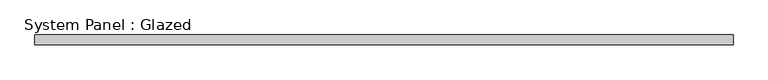
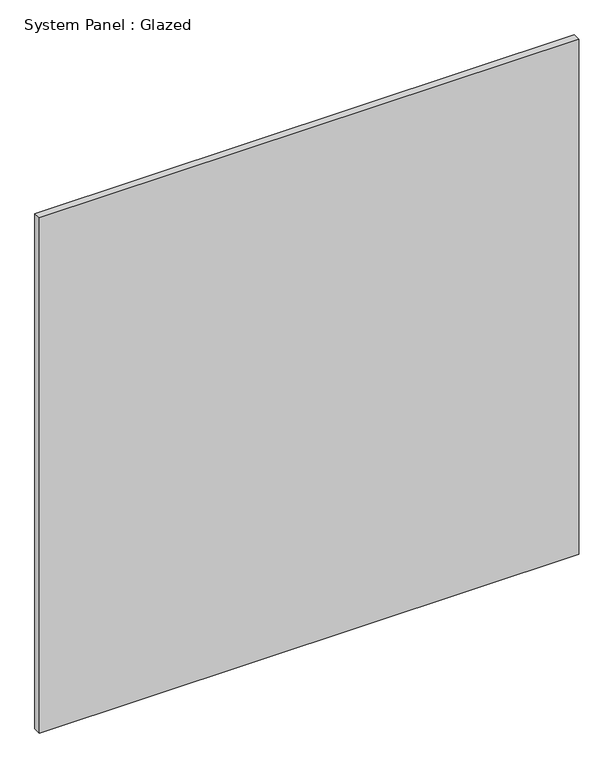
"""IFC4 building model written with IfcOpenShell, lengths in millimetres: plate geometry, System Panel : Glazed."""

from ifc_helpers import new_model, si_unit, origin, origin_with_axes, place, context, project, spatial, polyline, outline, extrude, source, transform, mapped, element, save


def system_panel_glazed_af581f75(model_context):
    return source(origin(), model_context, "Body", "SweptSolid", [
        extrude(outline(polyline([(877.5000002, 24.5), (-877.5000002, 24.5), (-877.5000002, 49.5), (877.5000002, 49.5), (877.5000002, 24.5)])), origin_with_axes(), (0.0, 0.0, 1.0), 1772.3836314),
    ])


if __name__ == "__main__":
    model = new_model("IFC4")
    model_context = context("Model", 3, world=origin())
    ifc_project = project(units=[si_unit("LENGTHUNIT", "METRE", prefix="MILLI")], contexts=[model_context])
    site = spatial("IfcSite", under=ifc_project)
    building = spatial("IfcBuilding", under=site)
    placement = place(None, origin())
    system_panel_glazed_shape = system_panel_glazed_af581f75(model_context)
    element("IfcPlate", 1, ObjectType="System Panel : Glazed", at=placement, inside=building, context=model_context, shape_type="MappedRepresentation", body=[
        mapped(system_panel_glazed_shape, transform((0.0, 0.0, 0.0), x_axis=(1.0, 0.0, 0.0), y_axis=(0.0, 1.0, 0.0), z_axis=(0.0, 0.0, 1.0))),
    ])
    save(model, "model.ifc")

# Revit data of these elements
# Element 1 (IfcPlate, "System Panel : Glazed")
#   Materials on its faces: "Glass"
# Materials
#   "Glass": class "Glass", colour RGB 218 227 224, transparency 0.85, Description = "Soda Lime Glass", Cost = 0
